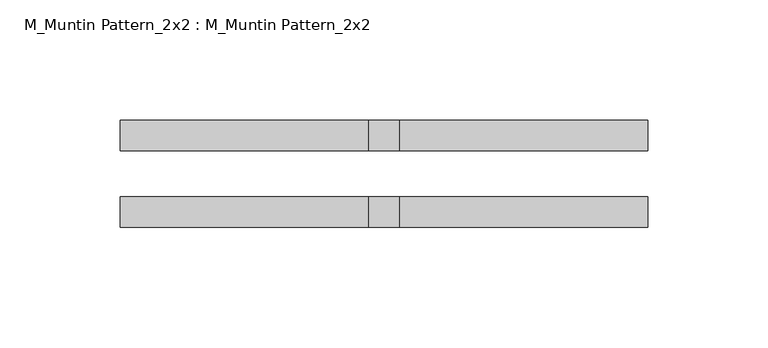
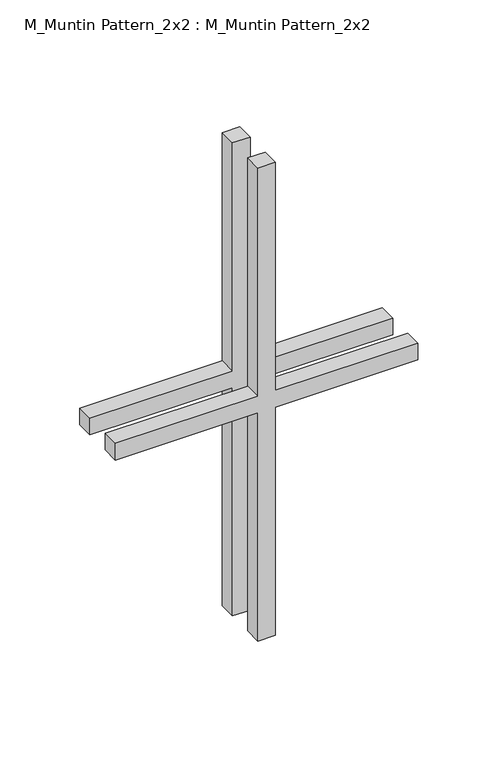
"""IFC4 building model written with IfcOpenShell, lengths in millimetres: proxy geometry, M_Muntin Pattern_2x2 : M_Muntin Pattern_2x2."""

import ifcopenshell
import ifcopenshell.guid

model = None  # the IFC model being written
_history = None  # IfcOwnerHistory: only IFC2X3 demands one
_inside = {}  # id of a spatial element -> (the spatial element, [elements in it])
_under = {}  # id of a project, library or spatial element -> (it, [spatial elements below it])
_declared = {}  # id of a project -> (the project, [libraries it declares])
_typed = {}  # id of a type object -> (the type object, [elements of that type])
_made_of = {}  # id of a material, layer set ... -> (it, [elements and type objects made of it])


def new_model(schema):
    """Start an empty IFC model of exactly this schema.

    Asked for "IFC4X3", IfcOpenShell would pick the latest addendum, in which some entities
    have other attributes; the version numbers below select the first issue.
    IFC2X3 requires an IfcOwnerHistory on every rooted entity: one is made here for all.
    """
    global model, _history
    if schema == "IFC4X3":
        model = ifcopenshell.file(schema_version=(4, 3, 0, 0))
    else:
        model = ifcopenshell.file(schema=schema)
    _inside.clear()
    _under.clear()
    _declared.clear()
    _typed.clear()
    _made_of.clear()
    _history = None
    if model.schema == "IFC2X3":
        org = make("IfcOrganization", Name="unknown")
        user = make(
            "IfcPersonAndOrganization",
            ThePerson=make("IfcPerson", FamilyName="unknown"),
            TheOrganization=org,
        )
        app = make(
            "IfcApplication",
            ApplicationDeveloper=org,
            Version="unknown",
            ApplicationFullName="unknown",
            ApplicationIdentifier="unknown",
        )
        _history = make(
            "IfcOwnerHistory",
            OwningUser=user,
            OwningApplication=app,
            ChangeAction="ADDED",
            CreationDate=0,
        )
    return model


def make(cls, **values):
    """One entity of the class cls with the attributes given. An attribute that is None is left unset."""
    return model.create_entity(
        cls, **{name: value for name, value in values.items() if value is not None}
    )


def rooted(cls, **values):
    """An entity with a GlobalId (a new one), such as an element, a storey or a relation."""
    return make(cls, GlobalId=ifcopenshell.guid.new(), OwnerHistory=_history, **values)


def si_unit(unit_type, name, prefix=None):
    """IfcSIUnit, for example si_unit("LENGTHUNIT", "METRE", prefix="MILLI")."""
    return make("IfcSIUnit", UnitType=unit_type, Prefix=prefix, Name=name)


def assignment(units):
    """IfcUnitAssignment: the units of a project."""
    return None if units is None else make("IfcUnitAssignment", Units=units)


def point(xyz):
    """IfcCartesianPoint."""
    return None if xyz is None else make("IfcCartesianPoint", Coordinates=xyz)


def direction(xyz):
    """IfcDirection."""
    return None if xyz is None else make("IfcDirection", DirectionRatios=xyz)


def frame(location, z_axis=None, x_axis=None):
    """IfcAxis2Placement3D, a coordinate frame: its origin and axes. An axis left out is left unset."""
    return make(
        "IfcAxis2Placement3D",
        Location=point(location),
        Axis=direction(z_axis),
        RefDirection=direction(x_axis),
    )


def origin():
    """The frame at (0, 0, 0) with its axes left unset."""
    return frame((0.0, 0.0, 0.0))


def place(relative_to, where):
    """IfcLocalPlacement: puts the frame where relative to a parent placement (None: the world)."""
    return make(
        "IfcLocalPlacement", PlacementRelTo=relative_to, RelativePlacement=where
    )


def context(
    kind, dimensions, precision=None, world=None, true_north=None, identifier=None
):
    """IfcGeometricRepresentationContext, for example the 3D "Model" context."""
    return make(
        "IfcGeometricRepresentationContext",
        ContextIdentifier=identifier,
        ContextType=kind,
        CoordinateSpaceDimension=dimensions,
        Precision=precision,
        WorldCoordinateSystem=world,
        TrueNorth=true_north,
    )


def project(units=None, contexts=None):
    """IfcProject with its units and contexts."""
    return rooted(
        "IfcProject",
        Name="project",
        RepresentationContexts=contexts,
        UnitsInContext=assignment(units),
    )


def spatial(cls, under=None, at=None, **own):
    """A site, building, storey or space (cls), placed at a placement, below another one or the project."""
    s = rooted(cls, ObjectPlacement=at, **own)
    if under is not None:
        _under.setdefault(under.id(), (under, []))[1].append(s)
    return s


def polyline(points):
    """IfcPolyline through the points."""
    return make("IfcPolyline", Points=[point(p) for p in points])


def outline(outer, holes=None, kind="AREA"):
    """IfcArbitraryClosedProfileDef: a profile drawn as a closed curve; with holes, ...WithVoids."""
    if holes is None:
        return make("IfcArbitraryClosedProfileDef", ProfileType=kind, OuterCurve=outer)
    return make(
        "IfcArbitraryProfileDefWithVoids",
        ProfileType=kind,
        OuterCurve=outer,
        InnerCurves=holes,
    )


def extrude(swept, where, along, depth):
    """IfcExtrudedAreaSolid: the profile swept, set in the frame where, extruded along a direction by depth."""
    return make(
        "IfcExtrudedAreaSolid",
        SweptArea=swept,
        Position=where,
        ExtrudedDirection=direction(along),
        Depth=depth,
    )


def shape(context_of_items, identifier, shape_type, items):
    """IfcShapeRepresentation: the items that make up one representation, for example the "Body"."""
    return make(
        "IfcShapeRepresentation",
        ContextOfItems=context_of_items,
        RepresentationIdentifier=identifier,
        RepresentationType=shape_type,
        Items=items,
    )


def source(mapping_origin, context_of_items, identifier, shape_type, items):
    """IfcRepresentationMap: a shape defined once, which mapped items show again and again."""
    return make(
        "IfcRepresentationMap",
        MappingOrigin=mapping_origin,
        MappedRepresentation=shape(context_of_items, identifier, shape_type, items),
    )


def transform(
    local_origin,
    x_axis=None,
    y_axis=None,
    z_axis=None,
    scale=None,
    scale2=None,
    scale3=None,
    uniform=True,
):
    """IfcCartesianTransformationOperator3D, or its non-uniform kind. x_axis, y_axis, z_axis: its Axis1, 2, 3."""
    if uniform:
        return make(
            "IfcCartesianTransformationOperator3D",
            Axis1=direction(x_axis),
            Axis2=direction(y_axis),
            LocalOrigin=point(local_origin),
            Scale=scale,
            Axis3=direction(z_axis),
        )
    return make(
        "IfcCartesianTransformationOperator3DnonUniform",
        Axis1=direction(x_axis),
        Axis2=direction(y_axis),
        LocalOrigin=point(local_origin),
        Scale=scale,
        Axis3=direction(z_axis),
        Scale2=scale2,
        Scale3=scale3,
    )


def mapped(mapping_source, mapping_target):
    """IfcMappedItem: shows the shape of a source again, moved by a transform."""
    return make(
        "IfcMappedItem", MappingSource=mapping_source, MappingTarget=mapping_target
    )


def made_of(thing, what):
    """Note that an element or type object is made of a material, layer set ...; save() writes the relation."""
    if what is not None:
        _made_of.setdefault(what.id(), (what, []))[1].append(thing)
    return thing


def element(
    cls,
    number,
    at=None,
    inside=None,
    cuts=None,
    type_object=None,
    material=None,
    context=None,
    identifier="Body",
    shape_type=None,
    held_by="IfcProductDefinitionShape",
    body=None,
    shapes=None,
    **own,
):
    """One element of the class cls, such as IfcWall. Its Tag is "e" and its number.

    at: its placement. inside: the storey or other place that contains it. cuts: it is an
    opening in that element (IfcRelVoidsElement). A single representation is given by context,
    identifier, shape_type and body (its items); several are given by shapes. held_by: the class
    of the entity that holds the representations. save() writes the other relations.
    """
    e = rooted(cls, Tag="e%d" % number, ObjectPlacement=at, **own)
    if body is not None:
        shapes = [shape(context, identifier, shape_type, body)]
    if shapes is not None:
        e.Representation = make(held_by, Representations=shapes)
    if inside is not None:
        _inside.setdefault(inside.id(), (inside, []))[1].append(e)
    if cuts is not None:
        rooted(
            "IfcRelVoidsElement", RelatingBuildingElement=cuts, RelatedOpeningElement=e
        )
    if type_object is not None:
        _typed.setdefault(type_object.id(), (type_object, []))[1].append(e)
    return made_of(e, material)


def aggregate(whole, parts):
    """IfcRelAggregates: a whole, such as a stair, and the parts it consists of."""
    return rooted("IfcRelAggregates", RelatingObject=whole, RelatedObjects=parts)


def save(model, path):
    """Write the relations noted so far, then the file.

    IfcRelAggregates (storeys below a building ...), IfcRelContainedInSpatialStructure (elements
    in a storey), IfcRelDefinesByType, IfcRelAssociatesMaterial and IfcRelDeclares: one each for
    every whole, place, type object, material and project.
    """
    for whole, parts in _under.values():
        aggregate(whole, parts)
    for where, things in _inside.values():
        rooted(
            "IfcRelContainedInSpatialStructure",
            RelatedElements=things,
            RelatingStructure=where,
        )
    for kind, things in _typed.values():
        rooted("IfcRelDefinesByType", RelatedObjects=things, RelatingType=kind)
    for what, things in _made_of.values():
        rooted("IfcRelAssociatesMaterial", RelatedObjects=things, RelatingMaterial=what)
    for by, libraries in _declared.values():
        rooted("IfcRelDeclares", RelatingContext=by, RelatedDefinitions=libraries)
    model.write(path)


def m_muntin_pattern_2x2_m_muntin_pattern_2x2_9617f888(model_context):
    return source(origin(), model_context, "Body", "SweptSolid", [
        extrude(outline(polyline([(187.325, -6.35), (187.325, -109.5375), (174.625, -109.5375), (174.625, -6.35), (0.0, -6.35), (0.0, 6.35), (174.625, 6.35), (174.625, 109.5375), (187.325, 109.5375), (187.325, 6.35), (361.95, 6.35), (361.95, -6.35), (187.325, -6.35)])), frame((0.0, -22.225, 0.0), z_axis=(0.0, 1.0, 0.0), x_axis=(0.0, 0.0, 1.0)), (0.0, 0.0, 1.0), 12.7),
        extrude(outline(polyline([(187.325, -6.35), (187.325, -109.5375), (174.625, -109.5375), (174.625, -6.35), (0.0, -6.35), (0.0, 6.35), (174.625, 6.35), (174.625, 109.5375), (187.325, 109.5375), (187.325, 6.35), (361.95, 6.35), (361.95, -6.35), (187.325, -6.35)])), frame((0.0, 9.525, 0.0), z_axis=(0.0, 1.0, 0.0), x_axis=(0.0, 0.0, 1.0)), (0.0, 0.0, 1.0), 12.7),
    ])


if __name__ == "__main__":
    model = new_model("IFC4")
    model_context = context("Model", 3, world=origin())
    ifc_project = project(units=[si_unit("LENGTHUNIT", "METRE", prefix="MILLI")], contexts=[model_context])
    site = spatial("IfcSite", under=ifc_project)
    building = spatial("IfcBuilding", under=site)
    placement = place(None, origin())
    m_muntin_pattern_2x2_m_muntin_pattern_2x2_shape = m_muntin_pattern_2x2_m_muntin_pattern_2x2_9617f888(model_context)
    element("IfcBuildingElementProxy", 1, Name="M_Muntin Pattern_2x2 : M_Muntin Pattern_2x2", ObjectType="M_Muntin Pattern_2x2 : M_Muntin Pattern_2x2", at=placement, inside=building, context=model_context, shape_type="MappedRepresentation", body=[
        mapped(m_muntin_pattern_2x2_m_muntin_pattern_2x2_shape, transform((0.0, 0.0, 0.0), x_axis=(1.0, 0.0, 0.0), y_axis=(0.0, 1.0, 0.0), z_axis=(0.0, 0.0, 1.0))),
    ])
    save(model, "model.ifc")

# Revit data of these elements
# Type "M_Muntin Pattern_2x2 : M_Muntin Pattern_2x2"
#   Width [instance default] = 3' - 11.24409"
#   Thickness = 0' - 0 1/2"
#   Height [instance default] = 3' - 11.24409"
#   Distance = 0' - 0 3/4"
#   Interior Material [instance default] = none
#   Exterior Material [instance default] = none
#   Default Elevation = 0
# Element 1 (IfcBuildingElementProxy, "M_Muntin Pattern_2x2 : M_Muntin Pattern_2x2")
#   Width = 0' - 8 5/8"
#   Height = 1' - 2 1/4"
#   Interior Material = Wood - Stained
#   Exterior Material = Clad - White
#   Materials on its faces: "Clad - White", "Wood - Stained"
# Materials
#   "Clad - White": class "Wood", colour RGB 242 242 238, transparency 0, Cost = 0
#   "Wood - Stained": class "Wood", colour RGB 224 178 126, transparency 0, Cost = 0
